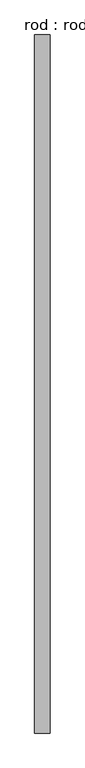
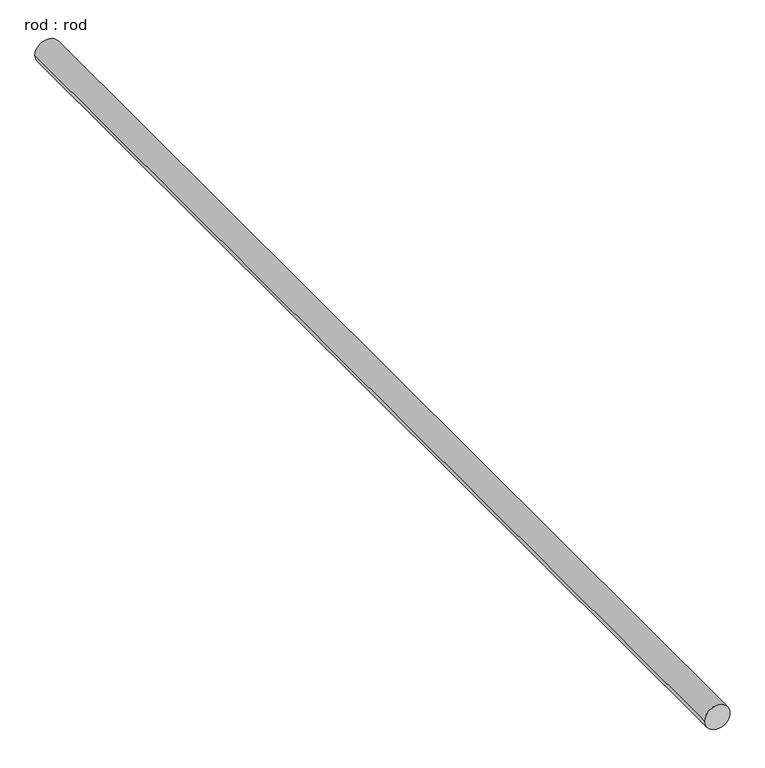
"""IFC4 building model written with IfcOpenShell, lengths in millimetres: proxy geometry, rod : rod."""

from ifc_helpers import new_model, si_unit, point, frame, frame_2d, origin, place, context, project, spatial, circle_curve, trimmed, segment, composite_curve, outline, extrude, source, transform, mapped, element, save


def rod_rod_4c2f9f54(model_context):
    return source(origin(), model_context, "Body", "SweptSolid", [
        extrude(outline(composite_curve([segment(trimmed(circle_curve(frame_2d((0.0108462, 0.0)), 200.0), [point((0.0108462, 200.0))], [point((0.0108462, -200.0))], False, "CARTESIAN"), True, "CONTINUOUS"), segment(trimmed(circle_curve(frame_2d((0.0108462, 0.0)), 200.0), [point((0.0108462, -200.0))], [point((0.0108462, 200.0))], False, "CARTESIAN"), True, "CONTINUOUS")], self_intersect=False)), frame((0.0, -5103.4704976, 0.0), z_axis=(0.0, 1.0, 0.0), x_axis=(0.0, 0.0, 1.0)), (0.0, 0.0, 1.0), 18392.3982259),
    ])


if __name__ == "__main__":
    model = new_model("IFC4")
    model_context = context("Model", 3, world=origin())
    ifc_project = project(units=[si_unit("LENGTHUNIT", "METRE", prefix="MILLI")], contexts=[model_context])
    site = spatial("IfcSite", under=ifc_project)
    building = spatial("IfcBuilding", under=site)
    placement = place(None, origin())
    rod_rod_shape = rod_rod_4c2f9f54(model_context)
    element("IfcBuildingElementProxy", 1, Name="rod : rod", ObjectType="rod : rod", at=placement, inside=building, context=model_context, shape_type="MappedRepresentation", body=[
        mapped(rod_rod_shape, transform((0.0, 0.0, 0.0), x_axis=(1.0, 0.0, 0.0), y_axis=(0.0, 1.0, 0.0), z_axis=(0.0, 0.0, 1.0))),
    ])
    save(model, "model.ifc")

# Revit data of these elements
# Type "rod : rod"
#   Default Elevation = 0
